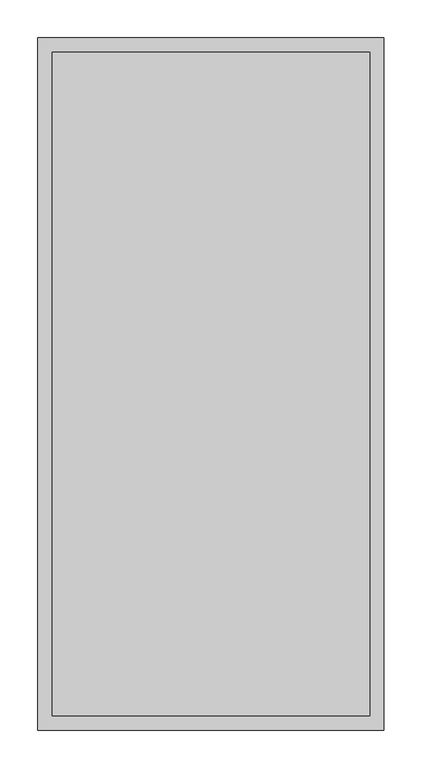
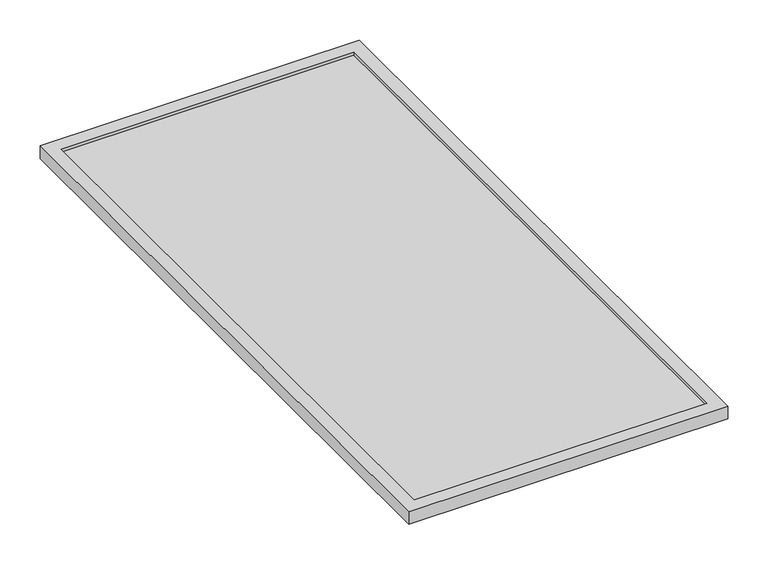
"""IFC4 building model written with IfcOpenShell, lengths in millimetres: proxy geometry, Bradley-Washroom_Accessories-Mirrors-780_Custom : Bradley-Washroom_Accessories-Mirrors-780_Custom."""

from ifc_helpers import new_model, si_unit, frame, origin, place, context, project, spatial, polyline, outline, extrude, faceted_brep, source, transform, mapped, element, save


def specialty_equipment_676f9192(model_context):
    return source(origin(), model_context, "Body", "SolidModel", [
        extrude(outline(polyline([(209.55, 438.15), (209.55, -438.15), (-209.55, -438.15), (-209.55, 438.15), (209.55, 438.15)])), frame((0.0, 0.0, 9.525), z_axis=(0.0, 0.0, 1.0), x_axis=(1.0, 0.0, 0.0)), (0.0, 0.0, 1.0), 4.7625),
        faceted_brep([(228.6, 457.2, 19.05), (-228.6, 457.2, 19.05), (-228.6, -457.2, 19.05), (228.6, -457.2, 19.05), (-209.55, 438.15, 19.05), (209.55, 438.15, 19.05), (209.55, -438.15, 19.05), (-209.55, -438.15, 19.05), (228.6, 457.2, 0.0), (228.6, -457.2, 0.0), (-228.6, -457.2, 0.0), (-228.6, 457.2, 0.0), (209.55, 438.15, 9.525), (-209.55, 438.15, 9.525), (-209.55, -438.15, 9.525), (209.55, -438.15, 9.525)], [[[0, 1, 2, 3], [4, 5, 6, 7]], [[8, 9, 10, 11]], [[1, 0, 8, 11]], [[2, 1, 11, 10]], [[3, 2, 10, 9]], [[0, 3, 9, 8]], [[12, 13, 14, 15]], [[13, 12, 5, 4]], [[14, 13, 4, 7]], [[15, 14, 7, 6]], [[12, 15, 6, 5]]]),
    ])


if __name__ == "__main__":
    model = new_model("IFC4")
    model_context = context("Model", 3, world=origin())
    ifc_project = project(units=[si_unit("LENGTHUNIT", "METRE", prefix="MILLI")], contexts=[model_context])
    site = spatial("IfcSite", under=ifc_project)
    building = spatial("IfcBuilding", under=site)
    placement = place(None, origin())
    specialty_equipment_shape = specialty_equipment_676f9192(model_context)
    element("IfcBuildingElementProxy", 1, Name="Bradley-Washroom_Accessories-Mirrors-780_Custom : Bradley-Washroom_Accessories-Mirrors-780_Custom", ObjectType="Bradley-Washroom_Accessories-Mirrors-780_Custom : Bradley-Washroom_Accessories-Mirrors-780_Custom", at=placement, inside=building, context=model_context, shape_type="MappedRepresentation", body=[
        mapped(specialty_equipment_shape, transform((0.0, 0.0, 0.0), x_axis=(1.0, 0.0, 0.0), y_axis=(0.0, 1.0, 0.0), z_axis=(0.0, 0.0, 1.0))),
    ])
    save(model, "model.ifc")

# Revit data of these elements
# Type "Bradley-Washroom_Accessories-Mirrors-780_Custom : Bradley-Washroom_Accessories-Mirrors-780_Custom"
#   Keynote = "M08831300.01"
#   Warranty Information = "Complete unit, excepting mirrors warranted for one year.\r\n Stainless steel mirror frames for fifteen years.\r\n Plate glass mirrors for fifteen years.\r\n This warranty does not cover installation or any other labor charges and does not apply to any units,\r\n which have been damaged by accident, abuse, improper installation, improper maintenance, or altered in any way."
#   Version = "1.0"
#   URL = "http://www.bradleycorp.com/"
#   Type Comments = "ERROR - If you are able to see this message you haven't loaded this  family correctly."
#   OmniClass Title = "Mirrors"
#   OmniClass Code = "23.40.95.17.17"
#   Modeling Code = ""
#   Model = "ERROR - If you are able to see this message you haven't loaded this  family correctly."
#   MasterFormat Title = "Commercial Toilet Accessories"
#   MasterFormat Number = "10 28 13. 13"
#   Manufacturer = "Bradley Corporation"
#   Industry Standards = "ASTM C 1036"
#   Fire Rating = "n/a"
#   Dimensional Limits [instance default] = "Either Width or Hight must be over 25\""
#   Description = "ERROR - If you are able to see this message you haven't loaded this  family correctly."
#   Copyright = "This Model Data is Property of Bradley Corporation"
#   Buy American Act = "Yes"
#   Assembly Code = "C1030900"
#   ADA Compliant = "Yes"
#   Width [instance default] = 1' - 6"
#   Total Width [instance default] = 1' - 6"
#   Total Height [instance default] = 3' - 0"
#   Height [instance default] = 3' - 0"
#   Depth [instance default] = 0' - 0 3/4"
#   Default Elevation = 3' - 4"
#   Reflective Material = Glass - Bradley Corp - BradEX - Polished Float Mirror
#   Frame Material = Bradley Corp Stainless Steel - Satin
# Element 1 (IfcBuildingElementProxy, "Bradley-Washroom_Accessories-Mirrors-780_Custom : Bradley-Washroom_Accessories-Mirrors-780_Custom")
#   Materials on its faces: "Bradley Corp Stainless Steel - Satin", "Glass - Bradley Corp - BradEX - Polished Float Mirror"
# Materials
#   "Glass - Bradley Corp - BradEX - Polished Float Mirror": class "Glass", colour RGB 221 230 232, transparency 0, Manufacturer = "Bradley Corporation", URL = "www.bradleycorp.com", Description = "Stainless Steel - Satin Finish", Cost = 0
#   "Bradley Corp Stainless Steel - Satin": class "Metal", colour RGB 189 187 185, transparency 0, Manufacturer = "Bradley Corporation", URL = "www.bradleycorp.com", Description = "Stainless Steel - Satin Finish", Cost = 0
